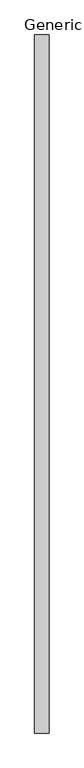
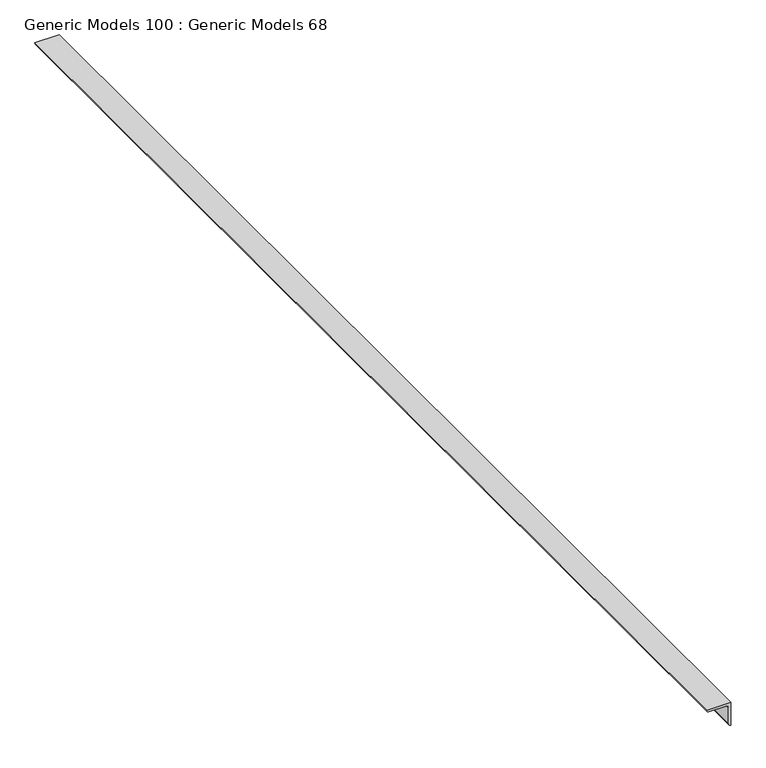
"""IFC4 building model written with IfcOpenShell, lengths in millimetres: proxy geometry, Generic Models 100 : Generic Models 68."""

from ifc_helpers import new_model, si_unit, point, frame, frame_2d, origin, place, context, project, spatial, polyline, circle_curve, trimmed, segment, composite_curve, outline, extrude, source, transform, mapped, element, save


def generic_models_100_generic_models_68_fff51ad1(model_context):
    return source(origin(), model_context, "Body", "SweptSolid", [
        extrude(outline(composite_curve([segment(polyline([(266004.6986952, 20503.9956945), (266004.6986952, 20440.4956945)]), True, "CONTINUOUS"), segment(trimmed(circle_curve(frame_2d((266004.6986952, 20446.8456945)), 6.35), [point((266004.6986952, 20440.4956945))], [point((265998.3486952, 20446.8456945))], False, "CARTESIAN"), True, "CONTINUOUS"), segment(polyline([(265998.3486952, 20446.8456945), (265998.3486952, 20491.2956945)]), True, "CONTINUOUS"), segment(trimmed(circle_curve(frame_2d((265991.9986952, 20491.2956945)), 6.35), [point((265998.3486952, 20491.2956945))], [point((265991.9986952, 20497.6456945))], True, "CARTESIAN"), True, "CONTINUOUS"), segment(polyline([(265991.9986952, 20497.6456945), (265947.5486952, 20497.6456945)]), True, "CONTINUOUS"), segment(trimmed(circle_curve(frame_2d((265947.5486952, 20503.9956945)), 6.35), [point((265947.5486952, 20497.6456945))], [point((265941.1986952, 20503.9956945))], False, "CARTESIAN"), True, "CONTINUOUS"), segment(polyline([(265941.1986952, 20503.9956945), (266004.6986952, 20503.9956945)]), True, "CONTINUOUS")], self_intersect=False)), frame((0.0, 18191.2264581, 0.0), z_axis=(0.0, 1.0, 0.0), x_axis=(0.0, 0.0, 1.0)), (0.0, 0.0, 1.0), 3048.0),
    ])


if __name__ == "__main__":
    model = new_model("IFC4")
    model_context = context("Model", 3, world=origin())
    ifc_project = project(units=[si_unit("LENGTHUNIT", "METRE", prefix="MILLI")], contexts=[model_context])
    site = spatial("IfcSite", under=ifc_project)
    building = spatial("IfcBuilding", under=site)
    placement = place(None, origin())
    generic_models_100_generic_models_68_shape = generic_models_100_generic_models_68_fff51ad1(model_context)
    element("IfcBuildingElementProxy", 1, Name="Generic Models 100 : Generic Models 68", ObjectType="Generic Models 100 : Generic Models 68", at=placement, inside=building, context=model_context, shape_type="MappedRepresentation", body=[
        mapped(generic_models_100_generic_models_68_shape, transform((0.0, 0.0, 0.0), x_axis=(1.0, 0.0, 0.0), y_axis=(0.0, 1.0, 0.0), z_axis=(0.0, 0.0, 1.0))),
    ])
    save(model, "model.ifc")

# Revit data of these elements
# Element 1 (IfcBuildingElementProxy, "Generic Models 100 : Generic Models 68")
#   Materials on its faces: "CAR DOOR RAIL: GALV. ANGLE L2 1/2 X 2 1/2 X 1/4\" @ 32\" ABOVE GRADE (PARALLEL TO HORTZ. WOOD TRIM)"
# Materials
#   "CAR DOOR RAIL: GALV. ANGLE L2 1/2 X 2 1/2 X 1/4\" @ 32\" ABOVE GRADE (PARALLEL TO HORTZ. WOOD TRIM)": class "Unassigned", colour RGB 211 211 211, transparency 0, Cost = 0
